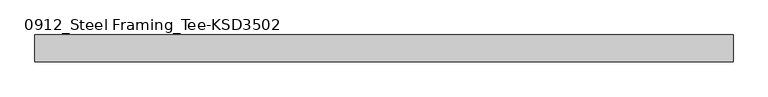
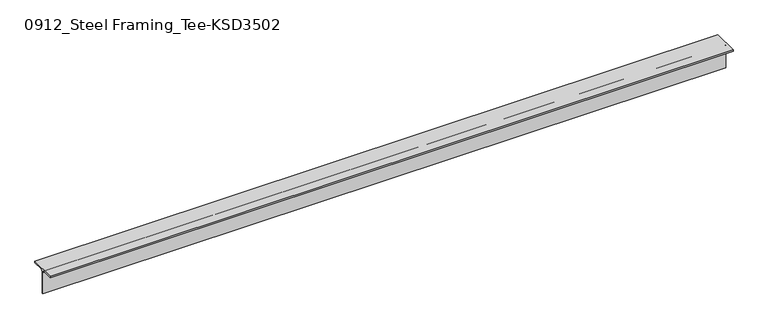
"""IFC4 building model written with IfcOpenShell, lengths in millimetres: member geometry, 0912_Steel Framing_Tee-KSD3502 : H_SB_ASB_CT-150x150x6.5x9."""

import ifcopenshell
import ifcopenshell.guid

model = None  # the IFC model being written
_history = None  # IfcOwnerHistory: only IFC2X3 demands one
_inside = {}  # id of a spatial element -> (the spatial element, [elements in it])
_under = {}  # id of a project, library or spatial element -> (it, [spatial elements below it])
_declared = {}  # id of a project -> (the project, [libraries it declares])
_typed = {}  # id of a type object -> (the type object, [elements of that type])
_made_of = {}  # id of a material, layer set ... -> (it, [elements and type objects made of it])


def new_model(schema):
    """Start an empty IFC model of exactly this schema.

    Asked for "IFC4X3", IfcOpenShell would pick the latest addendum, in which some entities
    have other attributes; the version numbers below select the first issue.
    IFC2X3 requires an IfcOwnerHistory on every rooted entity: one is made here for all.
    """
    global model, _history
    if schema == "IFC4X3":
        model = ifcopenshell.file(schema_version=(4, 3, 0, 0))
    else:
        model = ifcopenshell.file(schema=schema)
    _inside.clear()
    _under.clear()
    _declared.clear()
    _typed.clear()
    _made_of.clear()
    _history = None
    if model.schema == "IFC2X3":
        org = make("IfcOrganization", Name="unknown")
        user = make(
            "IfcPersonAndOrganization",
            ThePerson=make("IfcPerson", FamilyName="unknown"),
            TheOrganization=org,
        )
        app = make(
            "IfcApplication",
            ApplicationDeveloper=org,
            Version="unknown",
            ApplicationFullName="unknown",
            ApplicationIdentifier="unknown",
        )
        _history = make(
            "IfcOwnerHistory",
            OwningUser=user,
            OwningApplication=app,
            ChangeAction="ADDED",
            CreationDate=0,
        )
    return model


def make(cls, **values):
    """One entity of the class cls with the attributes given. An attribute that is None is left unset."""
    return model.create_entity(
        cls, **{name: value for name, value in values.items() if value is not None}
    )


def rooted(cls, **values):
    """An entity with a GlobalId (a new one), such as an element, a storey or a relation."""
    return make(cls, GlobalId=ifcopenshell.guid.new(), OwnerHistory=_history, **values)


def si_unit(unit_type, name, prefix=None):
    """IfcSIUnit, for example si_unit("LENGTHUNIT", "METRE", prefix="MILLI")."""
    return make("IfcSIUnit", UnitType=unit_type, Prefix=prefix, Name=name)


def assignment(units):
    """IfcUnitAssignment: the units of a project."""
    return None if units is None else make("IfcUnitAssignment", Units=units)


def point(xyz):
    """IfcCartesianPoint."""
    return None if xyz is None else make("IfcCartesianPoint", Coordinates=xyz)


def direction(xyz):
    """IfcDirection."""
    return None if xyz is None else make("IfcDirection", DirectionRatios=xyz)


def frame(location, z_axis=None, x_axis=None):
    """IfcAxis2Placement3D, a coordinate frame: its origin and axes. An axis left out is left unset."""
    return make(
        "IfcAxis2Placement3D",
        Location=point(location),
        Axis=direction(z_axis),
        RefDirection=direction(x_axis),
    )


def frame_2d(location, x_axis=None):
    """IfcAxis2Placement2D, a coordinate frame in the plane: its origin and x axis."""
    return make(
        "IfcAxis2Placement2D", Location=point(location), RefDirection=direction(x_axis)
    )


def origin():
    """The frame at (0, 0, 0) with its axes left unset."""
    return frame((0.0, 0.0, 0.0))


def place(relative_to, where):
    """IfcLocalPlacement: puts the frame where relative to a parent placement (None: the world)."""
    return make(
        "IfcLocalPlacement", PlacementRelTo=relative_to, RelativePlacement=where
    )


def context(
    kind, dimensions, precision=None, world=None, true_north=None, identifier=None
):
    """IfcGeometricRepresentationContext, for example the 3D "Model" context."""
    return make(
        "IfcGeometricRepresentationContext",
        ContextIdentifier=identifier,
        ContextType=kind,
        CoordinateSpaceDimension=dimensions,
        Precision=precision,
        WorldCoordinateSystem=world,
        TrueNorth=true_north,
    )


def project(units=None, contexts=None):
    """IfcProject with its units and contexts."""
    return rooted(
        "IfcProject",
        Name="project",
        RepresentationContexts=contexts,
        UnitsInContext=assignment(units),
    )


def spatial(cls, under=None, at=None, **own):
    """A site, building, storey or space (cls), placed at a placement, below another one or the project."""
    s = rooted(cls, ObjectPlacement=at, **own)
    if under is not None:
        _under.setdefault(under.id(), (under, []))[1].append(s)
    return s


def polyline(points):
    """IfcPolyline through the points."""
    return make("IfcPolyline", Points=[point(p) for p in points])


def circle_curve(where, radius):
    """IfcCircle in the frame where."""
    return make("IfcCircle", Position=where, Radius=radius)


def trimmed(basis, trim1, trim2, sense, master):
    """IfcTrimmedCurve: the piece of a basis curve between two trims."""
    return make(
        "IfcTrimmedCurve",
        BasisCurve=basis,
        Trim1=trim1,
        Trim2=trim2,
        SenseAgreement=sense,
        MasterRepresentation=master,
    )


def segment(curve, same_sense, transition):
    """IfcCompositeCurveSegment."""
    return make(
        "IfcCompositeCurveSegment",
        Transition=transition,
        SameSense=same_sense,
        ParentCurve=curve,
    )


def composite_curve(segments, self_intersect=None):
    """IfcCompositeCurve: segments joined end to end."""
    return make("IfcCompositeCurve", Segments=segments, SelfIntersect=self_intersect)


def outline(outer, holes=None, kind="AREA"):
    """IfcArbitraryClosedProfileDef: a profile drawn as a closed curve; with holes, ...WithVoids."""
    if holes is None:
        return make("IfcArbitraryClosedProfileDef", ProfileType=kind, OuterCurve=outer)
    return make(
        "IfcArbitraryProfileDefWithVoids",
        ProfileType=kind,
        OuterCurve=outer,
        InnerCurves=holes,
    )


def extrude(swept, where, along, depth):
    """IfcExtrudedAreaSolid: the profile swept, set in the frame where, extruded along a direction by depth."""
    return make(
        "IfcExtrudedAreaSolid",
        SweptArea=swept,
        Position=where,
        ExtrudedDirection=direction(along),
        Depth=depth,
    )


def shape(context_of_items, identifier, shape_type, items):
    """IfcShapeRepresentation: the items that make up one representation, for example the "Body"."""
    return make(
        "IfcShapeRepresentation",
        ContextOfItems=context_of_items,
        RepresentationIdentifier=identifier,
        RepresentationType=shape_type,
        Items=items,
    )


def source(mapping_origin, context_of_items, identifier, shape_type, items):
    """IfcRepresentationMap: a shape defined once, which mapped items show again and again."""
    return make(
        "IfcRepresentationMap",
        MappingOrigin=mapping_origin,
        MappedRepresentation=shape(context_of_items, identifier, shape_type, items),
    )


def transform(
    local_origin,
    x_axis=None,
    y_axis=None,
    z_axis=None,
    scale=None,
    scale2=None,
    scale3=None,
    uniform=True,
):
    """IfcCartesianTransformationOperator3D, or its non-uniform kind. x_axis, y_axis, z_axis: its Axis1, 2, 3."""
    if uniform:
        return make(
            "IfcCartesianTransformationOperator3D",
            Axis1=direction(x_axis),
            Axis2=direction(y_axis),
            LocalOrigin=point(local_origin),
            Scale=scale,
            Axis3=direction(z_axis),
        )
    return make(
        "IfcCartesianTransformationOperator3DnonUniform",
        Axis1=direction(x_axis),
        Axis2=direction(y_axis),
        LocalOrigin=point(local_origin),
        Scale=scale,
        Axis3=direction(z_axis),
        Scale2=scale2,
        Scale3=scale3,
    )


def mapped(mapping_source, mapping_target):
    """IfcMappedItem: shows the shape of a source again, moved by a transform."""
    return make(
        "IfcMappedItem", MappingSource=mapping_source, MappingTarget=mapping_target
    )


def made_of(thing, what):
    """Note that an element or type object is made of a material, layer set ...; save() writes the relation."""
    if what is not None:
        _made_of.setdefault(what.id(), (what, []))[1].append(thing)
    return thing


def element(
    cls,
    number,
    at=None,
    inside=None,
    cuts=None,
    type_object=None,
    material=None,
    context=None,
    identifier="Body",
    shape_type=None,
    held_by="IfcProductDefinitionShape",
    body=None,
    shapes=None,
    **own,
):
    """One element of the class cls, such as IfcWall. Its Tag is "e" and its number.

    at: its placement. inside: the storey or other place that contains it. cuts: it is an
    opening in that element (IfcRelVoidsElement). A single representation is given by context,
    identifier, shape_type and body (its items); several are given by shapes. held_by: the class
    of the entity that holds the representations. save() writes the other relations.
    """
    e = rooted(cls, Tag="e%d" % number, ObjectPlacement=at, **own)
    if body is not None:
        shapes = [shape(context, identifier, shape_type, body)]
    if shapes is not None:
        e.Representation = make(held_by, Representations=shapes)
    if inside is not None:
        _inside.setdefault(inside.id(), (inside, []))[1].append(e)
    if cuts is not None:
        rooted(
            "IfcRelVoidsElement", RelatingBuildingElement=cuts, RelatedOpeningElement=e
        )
    if type_object is not None:
        _typed.setdefault(type_object.id(), (type_object, []))[1].append(e)
    return made_of(e, material)


def aggregate(whole, parts):
    """IfcRelAggregates: a whole, such as a stair, and the parts it consists of."""
    return rooted("IfcRelAggregates", RelatingObject=whole, RelatedObjects=parts)


def save(model, path):
    """Write the relations noted so far, then the file.

    IfcRelAggregates (storeys below a building ...), IfcRelContainedInSpatialStructure (elements
    in a storey), IfcRelDefinesByType, IfcRelAssociatesMaterial and IfcRelDeclares: one each for
    every whole, place, type object, material and project.
    """
    for whole, parts in _under.values():
        aggregate(whole, parts)
    for where, things in _inside.values():
        rooted(
            "IfcRelContainedInSpatialStructure",
            RelatedElements=things,
            RelatingStructure=where,
        )
    for kind, things in _typed.values():
        rooted("IfcRelDefinesByType", RelatedObjects=things, RelatingType=kind)
    for what, things in _made_of.values():
        rooted("IfcRelAssociatesMaterial", RelatedObjects=things, RelatingMaterial=what)
    for by, libraries in _declared.values():
        rooted("IfcRelDeclares", RelatingContext=by, RelatedDefinitions=libraries)
    model.write(path)


def member_0912_steel_framing_tee_ksd3502_c81ff694(model_context):
    return source(origin(), model_context, "Body", "SweptSolid", [
        extrude(outline(composite_curve([segment(polyline([(-75.0, 75.0), (75.0, 75.0), (75.0, 66.0), (16.25, 66.0)]), True, "CONTINUOUS"), segment(trimmed(circle_curve(frame_2d((16.25, 53.0)), 13.0), [point((16.25, 66.0))], [point((3.25, 53.0))], True, "CARTESIAN"), True, "CONTINUOUS"), segment(polyline([(3.25, 53.0), (3.25, -75.0), (-3.25, -75.0), (-3.25, 53.0)]), True, "CONTINUOUS"), segment(trimmed(circle_curve(frame_2d((-16.25, 53.0)), 13.0), [point((-3.25, 53.0))], [point((-16.25, 66.0))], True, "CARTESIAN"), True, "CONTINUOUS"), segment(polyline([(-16.25, 66.0), (-75.0, 66.0), (-75.0, 75.0)]), True, "CONTINUOUS")], self_intersect=False)), frame((-1965.45, 0.0, 0.0), z_axis=(1.0, 0.0, 0.0), x_axis=(0.0, 1.0, 0.0)), (0.0, 0.0, 1.0), 3898.3),
    ])


if __name__ == "__main__":
    model = new_model("IFC4")
    model_context = context("Model", 3, world=origin())
    ifc_project = project(units=[si_unit("LENGTHUNIT", "METRE", prefix="MILLI")], contexts=[model_context])
    site = spatial("IfcSite", under=ifc_project)
    building = spatial("IfcBuilding", under=site)
    placement = place(None, origin())
    member_0912_steel_framing_tee_ksd3502_shape = member_0912_steel_framing_tee_ksd3502_c81ff694(model_context)
    element("IfcMember", 1, ObjectType="0912_Steel Framing_Tee-KSD3502 : H_SB_ASB_CT-150x150x6.5x9", at=placement, inside=building, context=model_context, shape_type="MappedRepresentation", body=[
        mapped(member_0912_steel_framing_tee_ksd3502_shape, transform((0.0, 0.0, 0.0), x_axis=(1.0, 0.0, 0.0), y_axis=(0.0, 1.0, 0.0), z_axis=(0.0, 0.0, 1.0))),
    ])
    save(model, "model.ifc")

# Revit data of these elements
# Type "0912_Steel Framing_Tee-KSD3502 : H_SB_ASB_CT-150x150x6.5x9"
#   H_WM Code_1 = "S01AA003-00001 | Main Steel Structure Fabrication Work | Shelter/Building | Light Steel - Standard (30KG/M>Weight) | Material: (   )"
#   H_WM Code_2 = "S03AA029-00001 | Main Steel Structure Erection Work | Shelter/Building | Light Steel (30KG/M>Weight) | Material: (   )"
#   H_WM Code_3 = "S01AA010-00001 | Main Steel Structure Fabrication Work | Shelter/Building | Steel Painting/Coating | for Non-Fireproofed Steel Surface, Surface Preparation, Primer, Second & Final Coat | Material: (   )"
#   H_Q'ty Cal Type Tag = "SB-Q2"
#   Width = 15.0 cm
#   Web Thickness = 0.65 cm
#   Web Fillet = 1.3 cm
#   Section Area = 23.39 cm²
#   Perimeter = 0.60 m²/m
#   Nominal Weight = 18.40 kgf/m
#   Height = 15.0 cm
#   Flange Thickness = 0.9 cm
#   Centroid Vertical = 7.5 cm
#   Centroid Horizontal = 7.5 cm
#   Length [instance default] = 1.5000 m
#   Structural Material [instance default] = Steel, 45-345
#   Warping Constant = (empty or 0)
#   Torsional Moment of Inertia = 0
#   Section Name Key = ""
#   Plastic Modulus weak axis = 0
#   Plastic Modulus strong axis = 0
#   Moment of Inertia weak axis = 0
#   Moment of Inertia strong axis = 0
#   Elastic Modulus weak axis = 0
#   Elastic Modulus strong axis = 0
#   Bolt Spacing = 0
#   Assembly Code = ""
# Element 1 (IfcMember, "0912_Steel Framing_Tee-KSD3502 : H_SB_ASB_CT-150x150x6.5x9")
#   Structural Material = none
# Materials
#   "Steel, 45-345": class "Metal", colour RGB 189 187 185, transparency 0, Description = "Steel 345 MPa", Cost = 0
